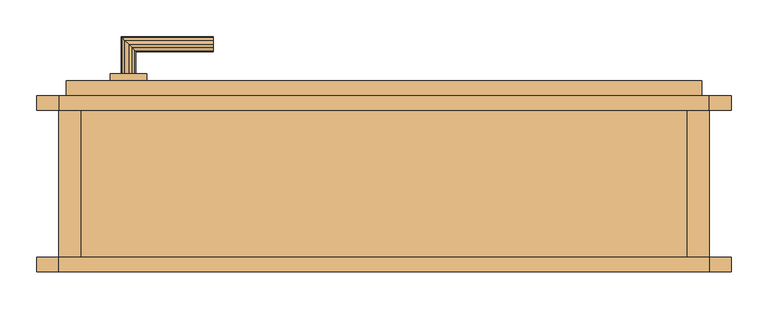
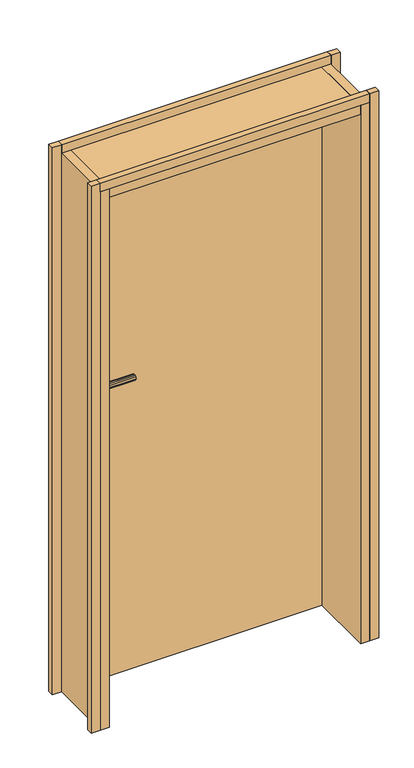
"""IFC4 building model written with IfcOpenShell, lengths in millimetres: door geometry, Tür."""

import ifcopenshell
import ifcopenshell.guid

model = None  # the IFC model being written
_history = None  # IfcOwnerHistory: only IFC2X3 demands one
_inside = {}  # id of a spatial element -> (the spatial element, [elements in it])
_under = {}  # id of a project, library or spatial element -> (it, [spatial elements below it])
_declared = {}  # id of a project -> (the project, [libraries it declares])
_typed = {}  # id of a type object -> (the type object, [elements of that type])
_made_of = {}  # id of a material, layer set ... -> (it, [elements and type objects made of it])


def new_model(schema):
    """Start an empty IFC model of exactly this schema.

    Asked for "IFC4X3", IfcOpenShell would pick the latest addendum, in which some entities
    have other attributes; the version numbers below select the first issue.
    IFC2X3 requires an IfcOwnerHistory on every rooted entity: one is made here for all.
    """
    global model, _history
    if schema == "IFC4X3":
        model = ifcopenshell.file(schema_version=(4, 3, 0, 0))
    else:
        model = ifcopenshell.file(schema=schema)
    _inside.clear()
    _under.clear()
    _declared.clear()
    _typed.clear()
    _made_of.clear()
    _history = None
    if model.schema == "IFC2X3":
        org = make("IfcOrganization", Name="unknown")
        user = make(
            "IfcPersonAndOrganization",
            ThePerson=make("IfcPerson", FamilyName="unknown"),
            TheOrganization=org,
        )
        app = make(
            "IfcApplication",
            ApplicationDeveloper=org,
            Version="unknown",
            ApplicationFullName="unknown",
            ApplicationIdentifier="unknown",
        )
        _history = make(
            "IfcOwnerHistory",
            OwningUser=user,
            OwningApplication=app,
            ChangeAction="ADDED",
            CreationDate=0,
        )
    return model


def make(cls, **values):
    """One entity of the class cls with the attributes given. An attribute that is None is left unset."""
    return model.create_entity(
        cls, **{name: value for name, value in values.items() if value is not None}
    )


def rooted(cls, **values):
    """An entity with a GlobalId (a new one), such as an element, a storey or a relation."""
    return make(cls, GlobalId=ifcopenshell.guid.new(), OwnerHistory=_history, **values)


def si_unit(unit_type, name, prefix=None):
    """IfcSIUnit, for example si_unit("LENGTHUNIT", "METRE", prefix="MILLI")."""
    return make("IfcSIUnit", UnitType=unit_type, Prefix=prefix, Name=name)


def assignment(units):
    """IfcUnitAssignment: the units of a project."""
    return None if units is None else make("IfcUnitAssignment", Units=units)


def point(xyz):
    """IfcCartesianPoint."""
    return None if xyz is None else make("IfcCartesianPoint", Coordinates=xyz)


def direction(xyz):
    """IfcDirection."""
    return None if xyz is None else make("IfcDirection", DirectionRatios=xyz)


def frame(location, z_axis=None, x_axis=None):
    """IfcAxis2Placement3D, a coordinate frame: its origin and axes. An axis left out is left unset."""
    return make(
        "IfcAxis2Placement3D",
        Location=point(location),
        Axis=direction(z_axis),
        RefDirection=direction(x_axis),
    )


def origin():
    """The frame at (0, 0, 0) with its axes left unset."""
    return frame((0.0, 0.0, 0.0))


def place(relative_to, where):
    """IfcLocalPlacement: puts the frame where relative to a parent placement (None: the world)."""
    return make(
        "IfcLocalPlacement", PlacementRelTo=relative_to, RelativePlacement=where
    )


def context(
    kind, dimensions, precision=None, world=None, true_north=None, identifier=None
):
    """IfcGeometricRepresentationContext, for example the 3D "Model" context."""
    return make(
        "IfcGeometricRepresentationContext",
        ContextIdentifier=identifier,
        ContextType=kind,
        CoordinateSpaceDimension=dimensions,
        Precision=precision,
        WorldCoordinateSystem=world,
        TrueNorth=true_north,
    )


def project(units=None, contexts=None):
    """IfcProject with its units and contexts."""
    return rooted(
        "IfcProject",
        Name="project",
        RepresentationContexts=contexts,
        UnitsInContext=assignment(units),
    )


def spatial(cls, under=None, at=None, **own):
    """A site, building, storey or space (cls), placed at a placement, below another one or the project."""
    s = rooted(cls, ObjectPlacement=at, **own)
    if under is not None:
        _under.setdefault(under.id(), (under, []))[1].append(s)
    return s


def polyline(points):
    """IfcPolyline through the points."""
    return make("IfcPolyline", Points=[point(p) for p in points])


def outline(outer, holes=None, kind="AREA"):
    """IfcArbitraryClosedProfileDef: a profile drawn as a closed curve; with holes, ...WithVoids."""
    if holes is None:
        return make("IfcArbitraryClosedProfileDef", ProfileType=kind, OuterCurve=outer)
    return make(
        "IfcArbitraryProfileDefWithVoids",
        ProfileType=kind,
        OuterCurve=outer,
        InnerCurves=holes,
    )


def extrude(swept, where, along, depth):
    """IfcExtrudedAreaSolid: the profile swept, set in the frame where, extruded along a direction by depth."""
    return make(
        "IfcExtrudedAreaSolid",
        SweptArea=swept,
        Position=where,
        ExtrudedDirection=direction(along),
        Depth=depth,
    )


def faces_of(points, faces, orient=None, outer=None):
    """IfcFace entities. A face is a list of loops; a loop is a list of indices into points, from 0.

    orient and outer hold one flag for each loop. By default every Orientation is true, the
    first loop of a face is its IfcFaceOuterBound and the others are IfcFaceBound.
    """
    made = []
    for i, loops in enumerate(faces):
        bounds = []
        for j, loop in enumerate(loops):
            is_outer = j == 0 if outer is None else outer[i][j]
            bounds.append(
                make(
                    "IfcFaceOuterBound" if is_outer else "IfcFaceBound",
                    Bound=make("IfcPolyLoop", Polygon=[points[k] for k in loop]),
                    Orientation=True if orient is None else orient[i][j],
                )
            )
        made.append(make("IfcFace", Bounds=bounds))
    return made


def faceted_brep(points, faces, orient=None, outer=None, voids=None):
    """IfcFacetedBrep: a solid bounded by flat faces; with voids (closed shells), ...WithVoids."""
    shared = [point(p) for p in points]
    hull = make("IfcClosedShell", CfsFaces=faces_of(shared, faces, orient, outer))
    if voids is None:
        return make("IfcFacetedBrep", Outer=hull)
    return make(
        "IfcFacetedBrepWithVoids",
        Outer=hull,
        Voids=[
            make(cls, CfsFaces=faces_of(shared, fs, o, b)) for cls, fs, o, b in voids
        ],
    )


def shape(context_of_items, identifier, shape_type, items):
    """IfcShapeRepresentation: the items that make up one representation, for example the "Body"."""
    return make(
        "IfcShapeRepresentation",
        ContextOfItems=context_of_items,
        RepresentationIdentifier=identifier,
        RepresentationType=shape_type,
        Items=items,
    )


def source(mapping_origin, context_of_items, identifier, shape_type, items):
    """IfcRepresentationMap: a shape defined once, which mapped items show again and again."""
    return make(
        "IfcRepresentationMap",
        MappingOrigin=mapping_origin,
        MappedRepresentation=shape(context_of_items, identifier, shape_type, items),
    )


def transform(
    local_origin,
    x_axis=None,
    y_axis=None,
    z_axis=None,
    scale=None,
    scale2=None,
    scale3=None,
    uniform=True,
):
    """IfcCartesianTransformationOperator3D, or its non-uniform kind. x_axis, y_axis, z_axis: its Axis1, 2, 3."""
    if uniform:
        return make(
            "IfcCartesianTransformationOperator3D",
            Axis1=direction(x_axis),
            Axis2=direction(y_axis),
            LocalOrigin=point(local_origin),
            Scale=scale,
            Axis3=direction(z_axis),
        )
    return make(
        "IfcCartesianTransformationOperator3DnonUniform",
        Axis1=direction(x_axis),
        Axis2=direction(y_axis),
        LocalOrigin=point(local_origin),
        Scale=scale,
        Axis3=direction(z_axis),
        Scale2=scale2,
        Scale3=scale3,
    )


def mapped(mapping_source, mapping_target):
    """IfcMappedItem: shows the shape of a source again, moved by a transform."""
    return make(
        "IfcMappedItem", MappingSource=mapping_source, MappingTarget=mapping_target
    )


def made_of(thing, what):
    """Note that an element or type object is made of a material, layer set ...; save() writes the relation."""
    if what is not None:
        _made_of.setdefault(what.id(), (what, []))[1].append(thing)
    return thing


def element(
    cls,
    number,
    at=None,
    inside=None,
    cuts=None,
    type_object=None,
    material=None,
    context=None,
    identifier="Body",
    shape_type=None,
    held_by="IfcProductDefinitionShape",
    body=None,
    shapes=None,
    **own,
):
    """One element of the class cls, such as IfcWall. Its Tag is "e" and its number.

    at: its placement. inside: the storey or other place that contains it. cuts: it is an
    opening in that element (IfcRelVoidsElement). A single representation is given by context,
    identifier, shape_type and body (its items); several are given by shapes. held_by: the class
    of the entity that holds the representations. save() writes the other relations.
    """
    e = rooted(cls, Tag="e%d" % number, ObjectPlacement=at, **own)
    if body is not None:
        shapes = [shape(context, identifier, shape_type, body)]
    if shapes is not None:
        e.Representation = make(held_by, Representations=shapes)
    if inside is not None:
        _inside.setdefault(inside.id(), (inside, []))[1].append(e)
    if cuts is not None:
        rooted(
            "IfcRelVoidsElement", RelatingBuildingElement=cuts, RelatedOpeningElement=e
        )
    if type_object is not None:
        _typed.setdefault(type_object.id(), (type_object, []))[1].append(e)
    return made_of(e, material)


def aggregate(whole, parts):
    """IfcRelAggregates: a whole, such as a stair, and the parts it consists of."""
    return rooted("IfcRelAggregates", RelatingObject=whole, RelatedObjects=parts)


def save(model, path):
    """Write the relations noted so far, then the file.

    IfcRelAggregates (storeys below a building ...), IfcRelContainedInSpatialStructure (elements
    in a storey), IfcRelDefinesByType, IfcRelAssociatesMaterial and IfcRelDeclares: one each for
    every whole, place, type object, material and project.
    """
    for whole, parts in _under.values():
        aggregate(whole, parts)
    for where, things in _inside.values():
        rooted(
            "IfcRelContainedInSpatialStructure",
            RelatedElements=things,
            RelatingStructure=where,
        )
    for kind, things in _typed.values():
        rooted("IfcRelDefinesByType", RelatedObjects=things, RelatingType=kind)
    for what, things in _made_of.values():
        rooted("IfcRelAssociatesMaterial", RelatedObjects=things, RelatingMaterial=what)
    for by, libraries in _declared.values():
        rooted("IfcRelDeclares", RelatingContext=by, RelatedDefinitions=libraries)
    model.write(path)


def door_c6220e3f(model_context):
    return source(origin(), model_context, "Body", "SolidModel", [
        extrude(outline(polyline([(885.0, -20.0), (0.0, -20.0), (0.0, 0.0), (885.0, 0.0), (885.0, -20.0)])), frame((0.0, 0.0, 2010.0), z_axis=(0.0, 0.0, 1.0), x_axis=(1.0, 0.0, 0.0)), (0.0, 0.0, 1.0), 30.0),
        extrude(outline(polyline([(0.0, -20.0), (-30.0, -20.0), (-30.0, 0.0), (0.0, 0.0), (0.0, -20.0)])), frame((0.0, 0.0, 140.0), z_axis=(0.0, 0.0, 1.0), x_axis=(1.0, 0.0, 0.0)), (0.0, 0.0, 1.0), 1900.0),
        extrude(outline(polyline([(885.0, -20.0), (855.0, -20.0), (855.0, 220.0), (885.0, 220.0), (885.0, -20.0)])), frame((0.0, 0.0, 140.0), z_axis=(0.0, 0.0, 1.0), x_axis=(1.0, 0.0, 0.0)), (0.0, 0.0, 1.0), 1870.0),
        extrude(outline(polyline([(70.0, 190.0), (70.0, 200.0), (120.0, 200.0), (120.0, 190.0), (70.0, 190.0)])), frame((0.0, 0.0, 1050.0), z_axis=(0.0, 0.0, 1.0), x_axis=(1.0, 0.0, 0.0)), (0.0, 0.0, 1.0), 215.0),
        faceted_brep([(90.0, 190.0, 1198.660254), (95.0, 190.0, 1200.0), (100.0, 190.0, 1198.660254), (103.660254, 190.0, 1195.0), (105.0, 190.0, 1190.0), (103.660254, 190.0, 1185.0), (100.0, 190.0, 1181.339746), (95.0, 190.0, 1180.0), (90.0, 190.0, 1181.339746), (86.339746, 190.0, 1185.0), (85.0, 190.0, 1190.0), (86.339746, 190.0, 1195.0), (95.0, 150.0, 1200.0), (90.0, 145.0, 1198.660254), (86.339746, 141.339746, 1195.0), (85.0, 140.0, 1190.0), (86.339746, 141.339746, 1185.0), (90.0, 145.0, 1181.339746), (95.0, 150.0, 1180.0), (100.0, 155.0, 1181.339746), (103.660254, 158.660254, 1185.0), (105.0, 160.0, 1190.0), (103.660254, 158.660254, 1195.0), (100.0, 155.0, 1198.660254), (210.0, 155.0, 1198.660254), (210.0, 150.0, 1200.0), (210.0, 145.0, 1198.660254), (210.0, 141.339746, 1195.0), (210.0, 140.0, 1190.0), (210.0, 141.339746, 1185.0), (210.0, 145.0, 1181.339746), (210.0, 150.0, 1180.0), (210.0, 155.0, 1181.339746), (210.0, 158.660254, 1185.0), (210.0, 160.0, 1190.0), (210.0, 158.660254, 1195.0)], [[[0, 1, 2, 3, 4, 5, 6, 7, 8, 9, 10, 11]], [[12, 1, 0, 13]], [[13, 0, 11, 14]], [[14, 11, 10, 15]], [[15, 10, 9, 16]], [[16, 9, 8, 17]], [[17, 8, 7, 18]], [[18, 7, 6, 19]], [[19, 6, 5, 20]], [[20, 5, 4, 21]], [[21, 4, 3, 22]], [[22, 3, 2, 23]], [[23, 2, 1, 12]], [[24, 25, 26, 27, 28, 29, 30, 31, 32, 33, 34, 35]], [[25, 12, 13, 26]], [[26, 13, 14, 27]], [[27, 14, 15, 28]], [[28, 15, 16, 29]], [[29, 16, 17, 30]], [[30, 17, 18, 31]], [[31, 18, 19, 32]], [[32, 19, 20, 33]], [[33, 20, 21, 34]], [[34, 21, 22, 35]], [[35, 22, 23, 24]], [[24, 23, 12, 25]]]),
        faceted_brep([(100.0, 250.0, 1198.660254), (95.0, 250.0, 1200.0), (90.0, 250.0, 1198.660254), (86.339746, 250.0, 1195.0), (85.0, 250.0, 1190.0), (86.339746, 250.0, 1185.0), (90.0, 250.0, 1181.339746), (95.0, 250.0, 1180.0), (100.0, 250.0, 1181.339746), (103.660254, 250.0, 1185.0), (105.0, 250.0, 1190.0), (103.660254, 250.0, 1195.0), (95.0, 290.0, 1200.0), (90.0, 295.0, 1198.660254), (86.339746, 298.660254, 1195.0), (85.0, 300.0, 1190.0), (86.339746, 298.660254, 1185.0), (90.0, 295.0, 1181.339746), (95.0, 290.0, 1180.0), (100.0, 285.0, 1181.339746), (103.660254, 281.339746, 1185.0), (105.0, 280.0, 1190.0), (103.660254, 281.339746, 1195.0), (100.0, 285.0, 1198.660254), (210.0, 295.0, 1198.660254), (210.0, 290.0, 1200.0), (210.0, 285.0, 1198.660254), (210.0, 281.339746, 1195.0), (210.0, 280.0, 1190.0), (210.0, 281.339746, 1185.0), (210.0, 285.0, 1181.339746), (210.0, 290.0, 1180.0), (210.0, 295.0, 1181.339746), (210.0, 298.660254, 1185.0), (210.0, 300.0, 1190.0), (210.0, 298.660254, 1195.0)], [[[0, 1, 2, 3, 4, 5, 6, 7, 8, 9, 10, 11]], [[2, 1, 12, 13]], [[3, 2, 13, 14]], [[4, 3, 14, 15]], [[5, 4, 15, 16]], [[6, 5, 16, 17]], [[7, 6, 17, 18]], [[8, 7, 18, 19]], [[9, 8, 19, 20]], [[10, 9, 20, 21]], [[11, 10, 21, 22]], [[0, 11, 22, 23]], [[1, 0, 23, 12]], [[24, 25, 26, 27, 28, 29, 30, 31, 32, 33, 34, 35]], [[13, 12, 25, 24]], [[14, 13, 24, 35]], [[15, 14, 35, 34]], [[16, 15, 34, 33]], [[17, 16, 33, 32]], [[18, 17, 32, 31]], [[19, 18, 31, 30]], [[20, 19, 30, 29]], [[21, 20, 29, 28]], [[22, 21, 28, 27]], [[23, 22, 27, 26]], [[12, 23, 26, 25]]]),
        extrude(outline(polyline([(0.0, 200.0), (-30.0, 200.0), (-30.0, 220.0), (0.0, 220.0), (0.0, 200.0)])), frame((0.0, 0.0, 140.0), z_axis=(0.0, 0.0, 1.0), x_axis=(1.0, 0.0, 0.0)), (0.0, 0.0, 1.0), 1900.0),
        extrude(outline(polyline([(120.0, 240.0), (70.0, 240.0), (70.0, 250.0), (120.0, 250.0), (120.0, 240.0)])), frame((0.0, 0.0, 1050.0), z_axis=(0.0, 0.0, 1.0), x_axis=(1.0, 0.0, 0.0)), (0.0, 0.0, 1.0), 215.0),
        extrude(outline(polyline([(30.0, -20.0), (0.0, -20.0), (0.0, 220.0), (30.0, 220.0), (30.0, -20.0)])), frame((0.0, 0.0, 140.0), z_axis=(0.0, 0.0, 1.0), x_axis=(1.0, 0.0, 0.0)), (0.0, 0.0, 1.0), 1870.0),
        extrude(outline(polyline([(915.0, 220.0), (915.0, 200.0), (885.0, 200.0), (885.0, 220.0), (915.0, 220.0)])), frame((0.0, 0.0, 140.0), z_axis=(0.0, 0.0, 1.0), x_axis=(1.0, 0.0, 0.0)), (0.0, 0.0, 1.0), 1900.0),
        extrude(outline(polyline([(915.0, 0.0), (915.0, -20.0), (885.0, -20.0), (885.0, 0.0), (915.0, 0.0)])), frame((0.0, 0.0, 140.0), z_axis=(0.0, 0.0, 1.0), x_axis=(1.0, 0.0, 0.0)), (0.0, 0.0, 1.0), 1900.0),
        extrude(outline(polyline([(855.0, -20.0), (30.0, -20.0), (30.0, 220.0), (855.0, 220.0), (855.0, -20.0)])), frame((0.0, 0.0, 1980.0), z_axis=(0.0, 0.0, 1.0), x_axis=(1.0, 0.0, 0.0)), (0.0, 0.0, 1.0), 30.0),
        extrude(outline(polyline([(885.0, 200.0), (0.0, 200.0), (0.0, 220.0), (885.0, 220.0), (885.0, 200.0)])), frame((0.0, 0.0, 2010.0), z_axis=(0.0, 0.0, 1.0), x_axis=(1.0, 0.0, 0.0)), (0.0, 0.0, 1.0), 30.0),
        extrude(outline(polyline([(875.0, 200.0), (10.0, 200.0), (10.0, 240.0), (875.0, 240.0), (875.0, 200.0)])), frame((0.0, 0.0, 140.0), z_axis=(0.0, 0.0, 1.0), x_axis=(1.0, 0.0, 0.0)), (0.0, 0.0, 1.0), 1860.0),
    ])


if __name__ == "__main__":
    model = new_model("IFC4")
    model_context = context("Model", 3, world=origin())
    ifc_project = project(units=[si_unit("LENGTHUNIT", "METRE", prefix="MILLI")], contexts=[model_context])
    site = spatial("IfcSite", under=ifc_project)
    building = spatial("IfcBuilding", under=site)
    placement = place(None, origin())
    door_shape = door_c6220e3f(model_context)
    element("IfcDoor", 1, ObjectType="Tür", at=placement, inside=building, context=model_context, shape_type="MappedRepresentation", body=[
        mapped(door_shape, transform((0.0, 0.0, 0.0), x_axis=(1.0, 0.0, 0.0), y_axis=(0.0, 1.0, 0.0), z_axis=(0.0, 0.0, 1.0))),
    ])
    save(model, "model.ifc")

# Revit data of these elements
# Type "Tür"
#   Type Mark = "32"
# Element 1 (IfcDoor, "Tür")
#   Materials on its faces: "tuer_beschlag", "tuer_holzzarge"
# Materials
#   "tuer_beschlag": class "Unassigned", colour RGB 128 128 128, transparency 0
#   "tuer_holzzarge": class "Unassigned", colour RGB 255 255 255, transparency 0
